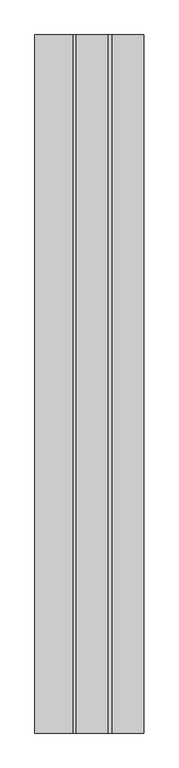
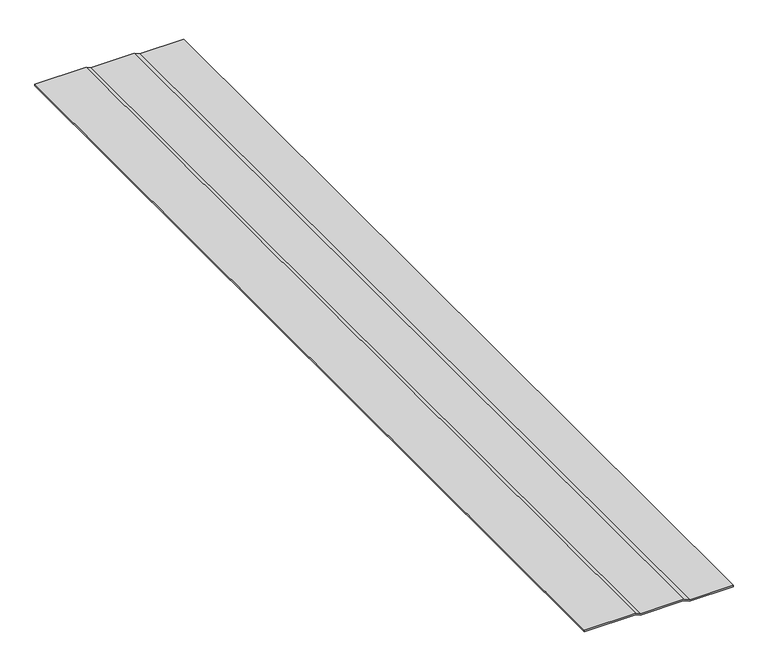
"""IFC4 building model written with IfcOpenShell, lengths in millimetres: proxy geometry, BITUMEN CAP SHEET003 14655 : BITUMEN CAP SHEET003 14655."""

from ifc_helpers import new_model, si_unit, frame, origin, place, context, project, spatial, polyline, outline, extrude, source, transform, mapped, element, save


def generic_models_03d49bda(model_context):
    return source(origin(), model_context, "Body", "SweptSolid", [
        extrude(outline(polyline([(40259.2002678, -2469.2761954), (40262.3752678, -2469.2761954), (40262.3752678, -2560.795457), (40267.6612773, -2573.2602756), (40267.6612773, -2663.9440313), (40271.9940719, -2673.6609328), (40271.9940719, -2781.5474293), (40268.8188423, -2781.5474293), (40268.8188423, -2674.3362183), (40264.4862773, -2664.6198318), (40264.4862773, -2573.9056756), (40259.2002678, -2561.440857), (40259.2002678, -2469.2761954)])), frame((0.0, 999.75, 0.0), z_axis=(0.0, 1.0, 0.0), x_axis=(0.0, 0.0, 1.0)), (0.0, 0.0, 1.0), 2000.25),
    ])


if __name__ == "__main__":
    model = new_model("IFC4")
    model_context = context("Model", 3, world=origin())
    ifc_project = project(units=[si_unit("LENGTHUNIT", "METRE", prefix="MILLI")], contexts=[model_context])
    site = spatial("IfcSite", under=ifc_project)
    building = spatial("IfcBuilding", under=site)
    placement = place(None, origin())
    generic_models_shape = generic_models_03d49bda(model_context)
    element("IfcBuildingElementProxy", 1, Name="BITUMEN CAP SHEET003 14655 : BITUMEN CAP SHEET003 14655", ObjectType="BITUMEN CAP SHEET003 14655 : BITUMEN CAP SHEET003 14655", at=placement, inside=building, context=model_context, shape_type="MappedRepresentation", body=[
        mapped(generic_models_shape, transform((0.0, 0.0, 0.0), x_axis=(1.0, 0.0, 0.0), y_axis=(0.0, 1.0, 0.0), z_axis=(0.0, 0.0, 1.0))),
    ])
    save(model, "model.ifc")

# Revit data of these elements
# Project information
#   Issued Date 1 = "0/00/2018 - City of Newport Beach"
#   IfcSite GUID = "3elgjS7H4HwQsE093rt3ko"
#   IfcBuilding GUID = "3eliBW7H4HwQsE093rt3ko"
#   IfcProject GUID = "3580753c_1e44_4e66_87a"
#   NameOverride = "Default Site"
#   Project Issue Date = "Issue Date"
#   Project Status = "Project Status"
#   Client Name = "xxx"
#   Project Address = "xxx"
#   Project Name = "STAUDENMEIER RESIDENCE"
# Type "BITUMEN CAP SHEET003 14655 : BITUMEN CAP SHEET003 14655"
#   NameOverride = "BITUMEN CAP SHEET003"
# Element 1 (IfcBuildingElementProxy, "BITUMEN CAP SHEET003 14655 : BITUMEN CAP SHEET003 14655")
#   Materials on its faces: "MODIFIED BITUMEN GRANULE SURFACED CAP SHEET"
# Materials
#   "MODIFIED BITUMEN GRANULE SURFACED CAP SHEET": class "Unassigned", colour RGB 85 85 127, transparency 0
